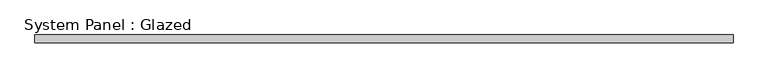
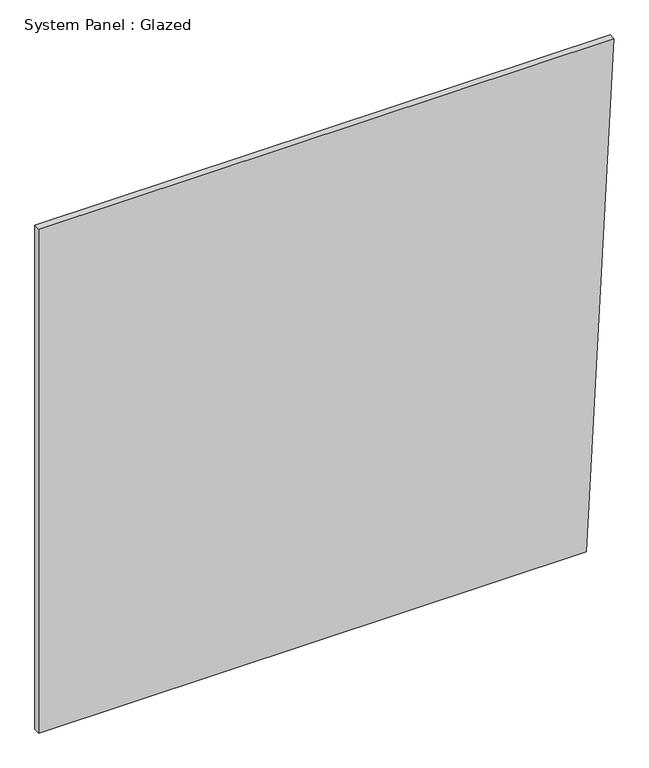
"""IFC4 building model written with IfcOpenShell, lengths in millimetres: plate geometry, System Panel : Glazed."""

import ifcopenshell
import ifcopenshell.guid

model = None  # the IFC model being written
_history = None  # IfcOwnerHistory: only IFC2X3 demands one
_inside = {}  # id of a spatial element -> (the spatial element, [elements in it])
_under = {}  # id of a project, library or spatial element -> (it, [spatial elements below it])
_declared = {}  # id of a project -> (the project, [libraries it declares])
_typed = {}  # id of a type object -> (the type object, [elements of that type])
_made_of = {}  # id of a material, layer set ... -> (it, [elements and type objects made of it])


def new_model(schema):
    """Start an empty IFC model of exactly this schema.

    Asked for "IFC4X3", IfcOpenShell would pick the latest addendum, in which some entities
    have other attributes; the version numbers below select the first issue.
    IFC2X3 requires an IfcOwnerHistory on every rooted entity: one is made here for all.
    """
    global model, _history
    if schema == "IFC4X3":
        model = ifcopenshell.file(schema_version=(4, 3, 0, 0))
    else:
        model = ifcopenshell.file(schema=schema)
    _inside.clear()
    _under.clear()
    _declared.clear()
    _typed.clear()
    _made_of.clear()
    _history = None
    if model.schema == "IFC2X3":
        org = make("IfcOrganization", Name="unknown")
        user = make(
            "IfcPersonAndOrganization",
            ThePerson=make("IfcPerson", FamilyName="unknown"),
            TheOrganization=org,
        )
        app = make(
            "IfcApplication",
            ApplicationDeveloper=org,
            Version="unknown",
            ApplicationFullName="unknown",
            ApplicationIdentifier="unknown",
        )
        _history = make(
            "IfcOwnerHistory",
            OwningUser=user,
            OwningApplication=app,
            ChangeAction="ADDED",
            CreationDate=0,
        )
    return model


def make(cls, **values):
    """One entity of the class cls with the attributes given. An attribute that is None is left unset."""
    return model.create_entity(
        cls, **{name: value for name, value in values.items() if value is not None}
    )


def rooted(cls, **values):
    """An entity with a GlobalId (a new one), such as an element, a storey or a relation."""
    return make(cls, GlobalId=ifcopenshell.guid.new(), OwnerHistory=_history, **values)


def si_unit(unit_type, name, prefix=None):
    """IfcSIUnit, for example si_unit("LENGTHUNIT", "METRE", prefix="MILLI")."""
    return make("IfcSIUnit", UnitType=unit_type, Prefix=prefix, Name=name)


def assignment(units):
    """IfcUnitAssignment: the units of a project."""
    return None if units is None else make("IfcUnitAssignment", Units=units)


def point(xyz):
    """IfcCartesianPoint."""
    return None if xyz is None else make("IfcCartesianPoint", Coordinates=xyz)


def direction(xyz):
    """IfcDirection."""
    return None if xyz is None else make("IfcDirection", DirectionRatios=xyz)


def frame(location, z_axis=None, x_axis=None):
    """IfcAxis2Placement3D, a coordinate frame: its origin and axes. An axis left out is left unset."""
    return make(
        "IfcAxis2Placement3D",
        Location=point(location),
        Axis=direction(z_axis),
        RefDirection=direction(x_axis),
    )


def origin():
    """The frame at (0, 0, 0) with its axes left unset."""
    return frame((0.0, 0.0, 0.0))


def place(relative_to, where):
    """IfcLocalPlacement: puts the frame where relative to a parent placement (None: the world)."""
    return make(
        "IfcLocalPlacement", PlacementRelTo=relative_to, RelativePlacement=where
    )


def context(
    kind, dimensions, precision=None, world=None, true_north=None, identifier=None
):
    """IfcGeometricRepresentationContext, for example the 3D "Model" context."""
    return make(
        "IfcGeometricRepresentationContext",
        ContextIdentifier=identifier,
        ContextType=kind,
        CoordinateSpaceDimension=dimensions,
        Precision=precision,
        WorldCoordinateSystem=world,
        TrueNorth=true_north,
    )


def project(units=None, contexts=None):
    """IfcProject with its units and contexts."""
    return rooted(
        "IfcProject",
        Name="project",
        RepresentationContexts=contexts,
        UnitsInContext=assignment(units),
    )


def spatial(cls, under=None, at=None, **own):
    """A site, building, storey or space (cls), placed at a placement, below another one or the project."""
    s = rooted(cls, ObjectPlacement=at, **own)
    if under is not None:
        _under.setdefault(under.id(), (under, []))[1].append(s)
    return s


def polyline(points):
    """IfcPolyline through the points."""
    return make("IfcPolyline", Points=[point(p) for p in points])


def outline(outer, holes=None, kind="AREA"):
    """IfcArbitraryClosedProfileDef: a profile drawn as a closed curve; with holes, ...WithVoids."""
    if holes is None:
        return make("IfcArbitraryClosedProfileDef", ProfileType=kind, OuterCurve=outer)
    return make(
        "IfcArbitraryProfileDefWithVoids",
        ProfileType=kind,
        OuterCurve=outer,
        InnerCurves=holes,
    )


def extrude(swept, where, along, depth):
    """IfcExtrudedAreaSolid: the profile swept, set in the frame where, extruded along a direction by depth."""
    return make(
        "IfcExtrudedAreaSolid",
        SweptArea=swept,
        Position=where,
        ExtrudedDirection=direction(along),
        Depth=depth,
    )


def shape(context_of_items, identifier, shape_type, items):
    """IfcShapeRepresentation: the items that make up one representation, for example the "Body"."""
    return make(
        "IfcShapeRepresentation",
        ContextOfItems=context_of_items,
        RepresentationIdentifier=identifier,
        RepresentationType=shape_type,
        Items=items,
    )


def source(mapping_origin, context_of_items, identifier, shape_type, items):
    """IfcRepresentationMap: a shape defined once, which mapped items show again and again."""
    return make(
        "IfcRepresentationMap",
        MappingOrigin=mapping_origin,
        MappedRepresentation=shape(context_of_items, identifier, shape_type, items),
    )


def transform(
    local_origin,
    x_axis=None,
    y_axis=None,
    z_axis=None,
    scale=None,
    scale2=None,
    scale3=None,
    uniform=True,
):
    """IfcCartesianTransformationOperator3D, or its non-uniform kind. x_axis, y_axis, z_axis: its Axis1, 2, 3."""
    if uniform:
        return make(
            "IfcCartesianTransformationOperator3D",
            Axis1=direction(x_axis),
            Axis2=direction(y_axis),
            LocalOrigin=point(local_origin),
            Scale=scale,
            Axis3=direction(z_axis),
        )
    return make(
        "IfcCartesianTransformationOperator3DnonUniform",
        Axis1=direction(x_axis),
        Axis2=direction(y_axis),
        LocalOrigin=point(local_origin),
        Scale=scale,
        Axis3=direction(z_axis),
        Scale2=scale2,
        Scale3=scale3,
    )


def mapped(mapping_source, mapping_target):
    """IfcMappedItem: shows the shape of a source again, moved by a transform."""
    return make(
        "IfcMappedItem", MappingSource=mapping_source, MappingTarget=mapping_target
    )


def made_of(thing, what):
    """Note that an element or type object is made of a material, layer set ...; save() writes the relation."""
    if what is not None:
        _made_of.setdefault(what.id(), (what, []))[1].append(thing)
    return thing


def element(
    cls,
    number,
    at=None,
    inside=None,
    cuts=None,
    type_object=None,
    material=None,
    context=None,
    identifier="Body",
    shape_type=None,
    held_by="IfcProductDefinitionShape",
    body=None,
    shapes=None,
    **own,
):
    """One element of the class cls, such as IfcWall. Its Tag is "e" and its number.

    at: its placement. inside: the storey or other place that contains it. cuts: it is an
    opening in that element (IfcRelVoidsElement). A single representation is given by context,
    identifier, shape_type and body (its items); several are given by shapes. held_by: the class
    of the entity that holds the representations. save() writes the other relations.
    """
    e = rooted(cls, Tag="e%d" % number, ObjectPlacement=at, **own)
    if body is not None:
        shapes = [shape(context, identifier, shape_type, body)]
    if shapes is not None:
        e.Representation = make(held_by, Representations=shapes)
    if inside is not None:
        _inside.setdefault(inside.id(), (inside, []))[1].append(e)
    if cuts is not None:
        rooted(
            "IfcRelVoidsElement", RelatingBuildingElement=cuts, RelatedOpeningElement=e
        )
    if type_object is not None:
        _typed.setdefault(type_object.id(), (type_object, []))[1].append(e)
    return made_of(e, material)


def aggregate(whole, parts):
    """IfcRelAggregates: a whole, such as a stair, and the parts it consists of."""
    return rooted("IfcRelAggregates", RelatingObject=whole, RelatedObjects=parts)


def save(model, path):
    """Write the relations noted so far, then the file.

    IfcRelAggregates (storeys below a building ...), IfcRelContainedInSpatialStructure (elements
    in a storey), IfcRelDefinesByType, IfcRelAssociatesMaterial and IfcRelDeclares: one each for
    every whole, place, type object, material and project.
    """
    for whole, parts in _under.values():
        aggregate(whole, parts)
    for where, things in _inside.values():
        rooted(
            "IfcRelContainedInSpatialStructure",
            RelatedElements=things,
            RelatingStructure=where,
        )
    for kind, things in _typed.values():
        rooted("IfcRelDefinesByType", RelatedObjects=things, RelatingType=kind)
    for what, things in _made_of.values():
        rooted("IfcRelAssociatesMaterial", RelatedObjects=things, RelatingMaterial=what)
    for by, libraries in _declared.values():
        rooted("IfcRelDeclares", RelatingContext=by, RelatedDefinitions=libraries)
    model.write(path)


def system_panel_glazed_3f2e0697(model_context):
    return source(origin(), model_context, "Body", "SweptSolid", [
        extrude(outline(polyline([(0.0, -1126.1853377), (0.0, 1017.0034845), (2086.1728929, 1126.1853377), (2086.1728929, -1126.1853377), (0.0, -1126.1853377)])), frame((0.0, -44.45, 0.0), z_axis=(0.0, 1.0, 0.0), x_axis=(0.0, 0.0, 1.0)), (0.0, 0.0, 1.0), 25.4),
    ])


if __name__ == "__main__":
    model = new_model("IFC4")
    model_context = context("Model", 3, world=origin())
    ifc_project = project(units=[si_unit("LENGTHUNIT", "METRE", prefix="MILLI")], contexts=[model_context])
    site = spatial("IfcSite", under=ifc_project)
    building = spatial("IfcBuilding", under=site)
    placement = place(None, origin())
    system_panel_glazed_shape = system_panel_glazed_3f2e0697(model_context)
    element("IfcPlate", 1, ObjectType="System Panel : Glazed", at=placement, inside=building, context=model_context, shape_type="MappedRepresentation", body=[
        mapped(system_panel_glazed_shape, transform((0.0, 0.0, 0.0), x_axis=(1.0, 0.0, 0.0), y_axis=(0.0, 1.0, 0.0), z_axis=(0.0, 0.0, 1.0))),
    ])
    save(model, "model.ifc")

# Revit data of these elements
# Type "System Panel : Glazed"
#   Construction Type Id = "GSP4R"
#   Analytic Construction = "1/8 in Pilkington single glazing"
#   Visual Light Transmittance = 0.9
#   Solar Heat Gain Coefficient = 0.86
#   Heat Transfer Coefficient (U) = 1.18115 BTU/(h·ft²·°F)
#   Define Thermal Properties by = 1
# Element 1 (IfcPlate, "System Panel : Glazed")
#   Materials on its faces: "Glass"
# Materials
#   "Glass": class "Glass", colour RGB 0 128 192, transparency 0.75, Description = "Soda Lime Glass", Cost = 0
